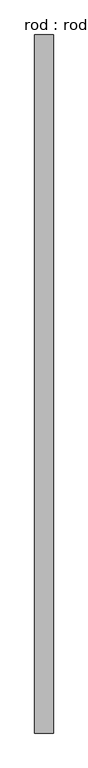
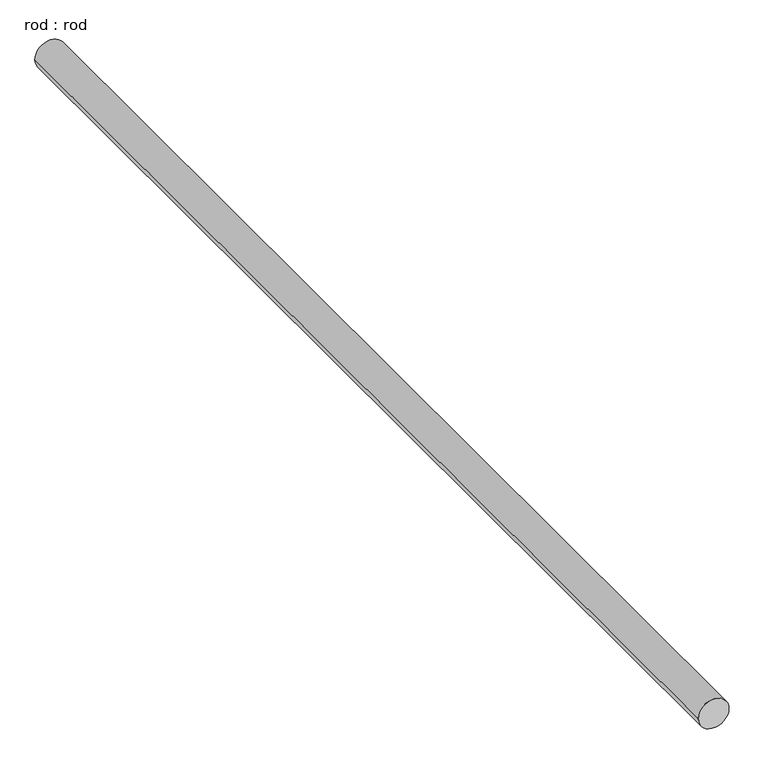
"""IFC4 building model written with IfcOpenShell, lengths in millimetres: proxy geometry, rod : rod."""

from ifc_helpers import new_model, si_unit, point, frame, frame_2d, origin, place, context, project, spatial, circle_curve, trimmed, segment, composite_curve, outline, extrude, source, transform, mapped, element, save


def rod_rod_78ed2e05(model_context):
    return source(origin(), model_context, "Body", "SweptSolid", [
        extrude(outline(composite_curve([segment(trimmed(circle_curve(frame_2d((0.0108462, 0.0)), 200.0), [point((0.0108462, 200.0))], [point((0.0108462, -200.0))], False, "CARTESIAN"), True, "CONTINUOUS"), segment(trimmed(circle_curve(frame_2d((0.0108462, 0.0)), 200.0), [point((0.0108462, -200.0))], [point((0.0108462, 200.0))], False, "CARTESIAN"), True, "CONTINUOUS")], self_intersect=False)), frame((0.0, -3393.8785275, 0.0), z_axis=(0.0, 1.0, 0.0), x_axis=(0.0, 0.0, 1.0)), (0.0, 0.0, 1.0), 14973.2142857),
    ])


if __name__ == "__main__":
    model = new_model("IFC4")
    model_context = context("Model", 3, world=origin())
    ifc_project = project(units=[si_unit("LENGTHUNIT", "METRE", prefix="MILLI")], contexts=[model_context])
    site = spatial("IfcSite", under=ifc_project)
    building = spatial("IfcBuilding", under=site)
    placement = place(None, origin())
    rod_rod_shape = rod_rod_78ed2e05(model_context)
    element("IfcBuildingElementProxy", 1, Name="rod : rod", ObjectType="rod : rod", at=placement, inside=building, context=model_context, shape_type="MappedRepresentation", body=[
        mapped(rod_rod_shape, transform((0.0, 0.0, 0.0), x_axis=(1.0, 0.0, 0.0), y_axis=(0.0, 1.0, 0.0), z_axis=(0.0, 0.0, 1.0))),
    ])
    save(model, "model.ifc")

# Revit data of these elements
# Type "rod : rod"
#   Default Elevation = 0
